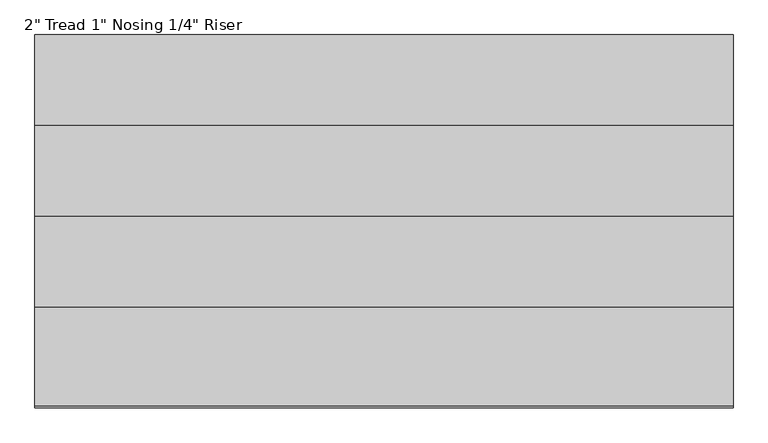
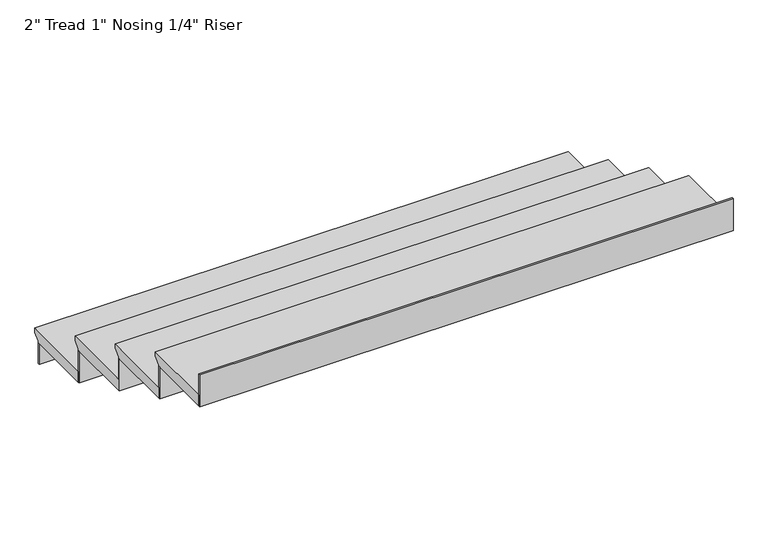
"""IFC4 building model written with IfcOpenShell, lengths in millimetres: stair flight geometry."""

from ifc_helpers import new_model, si_unit, frame, origin, place, context, project, spatial, polyline, outline, extrude, source, transform, mapped, element, save


def stair_flight_5efb7b33(model_context):
    return source(origin(), model_context, "Body", "SweptSolid", [
        extrude(outline(polyline([(18467.4054342, -613.8333333), (18797.6054342, -613.8333333), (18797.6054342, -632.8833333), (18772.2054342, -658.2833333), (18772.2054342, -664.6333333), (18467.4054342, -664.6333333), (18467.4054342, -613.8333333)])), frame((1099.2008381, 0.0, 0.0), z_axis=(1.0, 0.0, 0.0), x_axis=(0.0, 1.0, 0.0)), (0.0, 0.0, 1.0), 2338.1495078),
        extrude(outline(polyline([(1099.2008381, 18765.8554342), (1099.2008381, 18772.2054342), (3437.3503459, 18772.2054342), (3437.3503459, 18765.8554342), (1099.2008381, 18765.8554342)])), frame((0.0, 0.0, -762.0), z_axis=(0.0, 0.0, 1.0), x_axis=(1.0, 0.0, 0.0)), (0.0, 0.0, 1.0), 97.3666667),
        extrude(outline(polyline([(1099.2008381, 18461.0554342), (1099.2008381, 18467.4054342), (3437.3503459, 18467.4054342), (3437.3503459, 18461.0554342), (1099.2008381, 18461.0554342)])), frame((0.0, 0.0, -664.6333333), z_axis=(0.0, 0.0, 1.0), x_axis=(1.0, 0.0, 0.0)), (0.0, 0.0, 1.0), 148.1666667),
        extrude(outline(polyline([(18162.6054342, -465.6666667), (18492.8054342, -465.6666667), (18492.8054342, -484.7166667), (18467.4054342, -510.1166667), (18467.4054342, -516.4666667), (18162.6054342, -516.4666667), (18162.6054342, -465.6666667)])), frame((1099.2008381, 0.0, 0.0), z_axis=(1.0, 0.0, 0.0), x_axis=(0.0, 1.0, 0.0)), (0.0, 0.0, 1.0), 2338.1495078),
        extrude(outline(polyline([(1099.2008381, 18156.2554342), (1099.2008381, 18162.6054342), (3437.3503459, 18162.6054342), (3437.3503459, 18156.2554342), (1099.2008381, 18156.2554342)])), frame((0.0, 0.0, -516.4666667), z_axis=(0.0, 0.0, 1.0), x_axis=(1.0, 0.0, 0.0)), (0.0, 0.0, 1.0), 148.1666667),
        extrude(outline(polyline([(17857.8054342, -317.5), (18188.0054342, -317.5), (18188.0054342, -336.55), (18162.6054342, -361.95), (18162.6054342, -368.3), (17857.8054342, -368.3), (17857.8054342, -317.5)])), frame((1099.2008381, 0.0, 0.0), z_axis=(1.0, 0.0, 0.0), x_axis=(0.0, 1.0, 0.0)), (0.0, 0.0, 1.0), 2338.1495078),
        extrude(outline(polyline([(1099.2008381, 17851.4554342), (1099.2008381, 17857.8054342), (3437.3503459, 17857.8054342), (3437.3503459, 17851.4554342), (1099.2008381, 17851.4554342)])), frame((0.0, 0.0, -368.3), z_axis=(0.0, 0.0, 1.0), x_axis=(1.0, 0.0, 0.0)), (0.0, 0.0, 1.0), 148.1666667),
        extrude(outline(polyline([(1099.2008381, 17546.6554342), (1099.2008381, 17553.0054342), (3437.3503459, 17553.0054342), (3437.3503459, 17546.6554342), (1099.2008381, 17546.6554342)])), frame((0.0, 0.0, -220.1333333), z_axis=(0.0, 0.0, 1.0), x_axis=(1.0, 0.0, 0.0)), (0.0, 0.0, 1.0), 148.1666667),
        extrude(outline(polyline([(17553.0054342, -169.3333333), (17883.2054342, -169.3333333), (17883.2054342, -188.3833333), (17857.8054342, -213.7833333), (17857.8054342, -220.1333333), (17553.0054342, -220.1333333), (17553.0054342, -169.3333333)])), frame((1099.2008381, 0.0, 0.0), z_axis=(1.0, 0.0, 0.0), x_axis=(0.0, 1.0, 0.0)), (0.0, 0.0, 1.0), 2338.1495078),
    ])


if __name__ == "__main__":
    model = new_model("IFC4")
    model_context = context("Model", 3, world=origin())
    ifc_project = project(units=[si_unit("LENGTHUNIT", "METRE", prefix="MILLI")], contexts=[model_context])
    site = spatial("IfcSite", under=ifc_project)
    building = spatial("IfcBuilding", under=site)
    placement = place(None, origin())
    stair_flight_shape = stair_flight_5efb7b33(model_context)
    element("IfcStairFlight", 1, ObjectType="2\" Tread 1\" Nosing 1/4\" Riser", at=placement, inside=building, context=model_context, shape_type="MappedRepresentation", body=[
        mapped(stair_flight_shape, transform((0.0, 0.0, 0.0), x_axis=(1.0, 0.0, 0.0), y_axis=(0.0, 1.0, 0.0), z_axis=(0.0, 0.0, 1.0))),
    ])
    save(model, "model.ifc")
